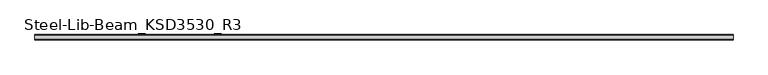
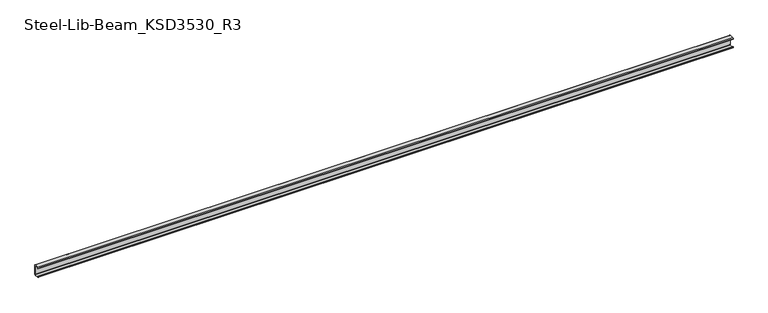
"""IFC4 building model written with IfcOpenShell, lengths in millimetres: beam geometry, Steel-Lib-Beam_KSD3530_R3 : BMS291_C-150×75x20x4.5."""

import ifcopenshell
import ifcopenshell.guid

model = None  # the IFC model being written
_history = None  # IfcOwnerHistory: only IFC2X3 demands one
_inside = {}  # id of a spatial element -> (the spatial element, [elements in it])
_under = {}  # id of a project, library or spatial element -> (it, [spatial elements below it])
_declared = {}  # id of a project -> (the project, [libraries it declares])
_typed = {}  # id of a type object -> (the type object, [elements of that type])
_made_of = {}  # id of a material, layer set ... -> (it, [elements and type objects made of it])


def new_model(schema):
    """Start an empty IFC model of exactly this schema.

    Asked for "IFC4X3", IfcOpenShell would pick the latest addendum, in which some entities
    have other attributes; the version numbers below select the first issue.
    IFC2X3 requires an IfcOwnerHistory on every rooted entity: one is made here for all.
    """
    global model, _history
    if schema == "IFC4X3":
        model = ifcopenshell.file(schema_version=(4, 3, 0, 0))
    else:
        model = ifcopenshell.file(schema=schema)
    _inside.clear()
    _under.clear()
    _declared.clear()
    _typed.clear()
    _made_of.clear()
    _history = None
    if model.schema == "IFC2X3":
        org = make("IfcOrganization", Name="unknown")
        user = make(
            "IfcPersonAndOrganization",
            ThePerson=make("IfcPerson", FamilyName="unknown"),
            TheOrganization=org,
        )
        app = make(
            "IfcApplication",
            ApplicationDeveloper=org,
            Version="unknown",
            ApplicationFullName="unknown",
            ApplicationIdentifier="unknown",
        )
        _history = make(
            "IfcOwnerHistory",
            OwningUser=user,
            OwningApplication=app,
            ChangeAction="ADDED",
            CreationDate=0,
        )
    return model


def make(cls, **values):
    """One entity of the class cls with the attributes given. An attribute that is None is left unset."""
    return model.create_entity(
        cls, **{name: value for name, value in values.items() if value is not None}
    )


def rooted(cls, **values):
    """An entity with a GlobalId (a new one), such as an element, a storey or a relation."""
    return make(cls, GlobalId=ifcopenshell.guid.new(), OwnerHistory=_history, **values)


def si_unit(unit_type, name, prefix=None):
    """IfcSIUnit, for example si_unit("LENGTHUNIT", "METRE", prefix="MILLI")."""
    return make("IfcSIUnit", UnitType=unit_type, Prefix=prefix, Name=name)


def assignment(units):
    """IfcUnitAssignment: the units of a project."""
    return None if units is None else make("IfcUnitAssignment", Units=units)


def point(xyz):
    """IfcCartesianPoint."""
    return None if xyz is None else make("IfcCartesianPoint", Coordinates=xyz)


def direction(xyz):
    """IfcDirection."""
    return None if xyz is None else make("IfcDirection", DirectionRatios=xyz)


def frame(location, z_axis=None, x_axis=None):
    """IfcAxis2Placement3D, a coordinate frame: its origin and axes. An axis left out is left unset."""
    return make(
        "IfcAxis2Placement3D",
        Location=point(location),
        Axis=direction(z_axis),
        RefDirection=direction(x_axis),
    )


def frame_2d(location, x_axis=None):
    """IfcAxis2Placement2D, a coordinate frame in the plane: its origin and x axis."""
    return make(
        "IfcAxis2Placement2D", Location=point(location), RefDirection=direction(x_axis)
    )


def origin():
    """The frame at (0, 0, 0) with its axes left unset."""
    return frame((0.0, 0.0, 0.0))


def place(relative_to, where):
    """IfcLocalPlacement: puts the frame where relative to a parent placement (None: the world)."""
    return make(
        "IfcLocalPlacement", PlacementRelTo=relative_to, RelativePlacement=where
    )


def context(
    kind, dimensions, precision=None, world=None, true_north=None, identifier=None
):
    """IfcGeometricRepresentationContext, for example the 3D "Model" context."""
    return make(
        "IfcGeometricRepresentationContext",
        ContextIdentifier=identifier,
        ContextType=kind,
        CoordinateSpaceDimension=dimensions,
        Precision=precision,
        WorldCoordinateSystem=world,
        TrueNorth=true_north,
    )


def project(units=None, contexts=None):
    """IfcProject with its units and contexts."""
    return rooted(
        "IfcProject",
        Name="project",
        RepresentationContexts=contexts,
        UnitsInContext=assignment(units),
    )


def spatial(cls, under=None, at=None, **own):
    """A site, building, storey or space (cls), placed at a placement, below another one or the project."""
    s = rooted(cls, ObjectPlacement=at, **own)
    if under is not None:
        _under.setdefault(under.id(), (under, []))[1].append(s)
    return s


def polyline(points):
    """IfcPolyline through the points."""
    return make("IfcPolyline", Points=[point(p) for p in points])


def circle_curve(where, radius):
    """IfcCircle in the frame where."""
    return make("IfcCircle", Position=where, Radius=radius)


def trimmed(basis, trim1, trim2, sense, master):
    """IfcTrimmedCurve: the piece of a basis curve between two trims."""
    return make(
        "IfcTrimmedCurve",
        BasisCurve=basis,
        Trim1=trim1,
        Trim2=trim2,
        SenseAgreement=sense,
        MasterRepresentation=master,
    )


def segment(curve, same_sense, transition):
    """IfcCompositeCurveSegment."""
    return make(
        "IfcCompositeCurveSegment",
        Transition=transition,
        SameSense=same_sense,
        ParentCurve=curve,
    )


def composite_curve(segments, self_intersect=None):
    """IfcCompositeCurve: segments joined end to end."""
    return make("IfcCompositeCurve", Segments=segments, SelfIntersect=self_intersect)


def outline(outer, holes=None, kind="AREA"):
    """IfcArbitraryClosedProfileDef: a profile drawn as a closed curve; with holes, ...WithVoids."""
    if holes is None:
        return make("IfcArbitraryClosedProfileDef", ProfileType=kind, OuterCurve=outer)
    return make(
        "IfcArbitraryProfileDefWithVoids",
        ProfileType=kind,
        OuterCurve=outer,
        InnerCurves=holes,
    )


def extrude(swept, where, along, depth):
    """IfcExtrudedAreaSolid: the profile swept, set in the frame where, extruded along a direction by depth."""
    return make(
        "IfcExtrudedAreaSolid",
        SweptArea=swept,
        Position=where,
        ExtrudedDirection=direction(along),
        Depth=depth,
    )


def shape(context_of_items, identifier, shape_type, items):
    """IfcShapeRepresentation: the items that make up one representation, for example the "Body"."""
    return make(
        "IfcShapeRepresentation",
        ContextOfItems=context_of_items,
        RepresentationIdentifier=identifier,
        RepresentationType=shape_type,
        Items=items,
    )


def source(mapping_origin, context_of_items, identifier, shape_type, items):
    """IfcRepresentationMap: a shape defined once, which mapped items show again and again."""
    return make(
        "IfcRepresentationMap",
        MappingOrigin=mapping_origin,
        MappedRepresentation=shape(context_of_items, identifier, shape_type, items),
    )


def transform(
    local_origin,
    x_axis=None,
    y_axis=None,
    z_axis=None,
    scale=None,
    scale2=None,
    scale3=None,
    uniform=True,
):
    """IfcCartesianTransformationOperator3D, or its non-uniform kind. x_axis, y_axis, z_axis: its Axis1, 2, 3."""
    if uniform:
        return make(
            "IfcCartesianTransformationOperator3D",
            Axis1=direction(x_axis),
            Axis2=direction(y_axis),
            LocalOrigin=point(local_origin),
            Scale=scale,
            Axis3=direction(z_axis),
        )
    return make(
        "IfcCartesianTransformationOperator3DnonUniform",
        Axis1=direction(x_axis),
        Axis2=direction(y_axis),
        LocalOrigin=point(local_origin),
        Scale=scale,
        Axis3=direction(z_axis),
        Scale2=scale2,
        Scale3=scale3,
    )


def mapped(mapping_source, mapping_target):
    """IfcMappedItem: shows the shape of a source again, moved by a transform."""
    return make(
        "IfcMappedItem", MappingSource=mapping_source, MappingTarget=mapping_target
    )


def made_of(thing, what):
    """Note that an element or type object is made of a material, layer set ...; save() writes the relation."""
    if what is not None:
        _made_of.setdefault(what.id(), (what, []))[1].append(thing)
    return thing


def element(
    cls,
    number,
    at=None,
    inside=None,
    cuts=None,
    type_object=None,
    material=None,
    context=None,
    identifier="Body",
    shape_type=None,
    held_by="IfcProductDefinitionShape",
    body=None,
    shapes=None,
    **own,
):
    """One element of the class cls, such as IfcWall. Its Tag is "e" and its number.

    at: its placement. inside: the storey or other place that contains it. cuts: it is an
    opening in that element (IfcRelVoidsElement). A single representation is given by context,
    identifier, shape_type and body (its items); several are given by shapes. held_by: the class
    of the entity that holds the representations. save() writes the other relations.
    """
    e = rooted(cls, Tag="e%d" % number, ObjectPlacement=at, **own)
    if body is not None:
        shapes = [shape(context, identifier, shape_type, body)]
    if shapes is not None:
        e.Representation = make(held_by, Representations=shapes)
    if inside is not None:
        _inside.setdefault(inside.id(), (inside, []))[1].append(e)
    if cuts is not None:
        rooted(
            "IfcRelVoidsElement", RelatingBuildingElement=cuts, RelatedOpeningElement=e
        )
    if type_object is not None:
        _typed.setdefault(type_object.id(), (type_object, []))[1].append(e)
    return made_of(e, material)


def aggregate(whole, parts):
    """IfcRelAggregates: a whole, such as a stair, and the parts it consists of."""
    return rooted("IfcRelAggregates", RelatingObject=whole, RelatedObjects=parts)


def save(model, path):
    """Write the relations noted so far, then the file.

    IfcRelAggregates (storeys below a building ...), IfcRelContainedInSpatialStructure (elements
    in a storey), IfcRelDefinesByType, IfcRelAssociatesMaterial and IfcRelDeclares: one each for
    every whole, place, type object, material and project.
    """
    for whole, parts in _under.values():
        aggregate(whole, parts)
    for where, things in _inside.values():
        rooted(
            "IfcRelContainedInSpatialStructure",
            RelatedElements=things,
            RelatingStructure=where,
        )
    for kind, things in _typed.values():
        rooted("IfcRelDefinesByType", RelatedObjects=things, RelatingType=kind)
    for what, things in _made_of.values():
        rooted("IfcRelAssociatesMaterial", RelatedObjects=things, RelatingMaterial=what)
    for by, libraries in _declared.values():
        rooted("IfcRelDeclares", RelatingContext=by, RelatedDefinitions=libraries)
    model.write(path)


def steel_lib_beam_ksd3530_r3_103558c8(model_context):
    return source(origin(), model_context, "Body", "SweptSolid", [
        extrude(outline(composite_curve([segment(trimmed(circle_curve(frame_2d((-41.0, 66.0)), 9.0), [point((-50.0, 66.0))], [point((-41.0, 75.0))], False, "CARTESIAN"), True, "CONTINUOUS"), segment(polyline([(-41.0, 75.0), (16.0, 75.0)]), True, "CONTINUOUS"), segment(trimmed(circle_curve(frame_2d((16.0, 66.0)), 9.0), [point((16.0, 75.0))], [point((25.0, 66.0))], False, "CARTESIAN"), True, "CONTINUOUS"), segment(polyline([(25.0, 66.0), (25.0, -66.0)]), True, "CONTINUOUS"), segment(trimmed(circle_curve(frame_2d((16.0, -66.0)), 9.0), [point((25.0, -66.0))], [point((16.0, -75.0))], False, "CARTESIAN"), True, "CONTINUOUS"), segment(polyline([(16.0, -75.0), (-41.0, -75.0)]), True, "CONTINUOUS"), segment(trimmed(circle_curve(frame_2d((-41.0, -66.0)), 9.0), [point((-41.0, -75.0))], [point((-50.0, -66.0))], False, "CARTESIAN"), True, "CONTINUOUS"), segment(polyline([(-50.0, -66.0), (-50.0, -55.0), (-45.5, -55.0), (-45.5, -66.0)]), True, "CONTINUOUS"), segment(trimmed(circle_curve(frame_2d((-41.0, -66.0)), 4.5), [point((-45.5, -66.0))], [point((-41.0, -70.5))], True, "CARTESIAN"), True, "CONTINUOUS"), segment(polyline([(-41.0, -70.5), (16.0, -70.5)]), True, "CONTINUOUS"), segment(trimmed(circle_curve(frame_2d((16.0, -66.0)), 4.5), [point((16.0, -70.5))], [point((20.5, -66.0))], True, "CARTESIAN"), True, "CONTINUOUS"), segment(polyline([(20.5, -66.0), (20.5, 66.0)]), True, "CONTINUOUS"), segment(trimmed(circle_curve(frame_2d((16.0, 66.0)), 4.5), [point((20.5, 66.0))], [point((16.0, 70.5))], True, "CARTESIAN"), True, "CONTINUOUS"), segment(polyline([(16.0, 70.5), (-41.0, 70.5)]), True, "CONTINUOUS"), segment(trimmed(circle_curve(frame_2d((-41.0, 66.0)), 4.5), [point((-41.0, 70.5))], [point((-45.5, 66.0))], True, "CARTESIAN"), True, "CONTINUOUS"), segment(polyline([(-45.5, 66.0), (-45.5, 55.0), (-50.0, 55.0), (-50.0, 66.0)]), True, "CONTINUOUS")], self_intersect=False)), frame((-4752.0, 0.0, 0.0), z_axis=(1.0, 0.0, 0.0), x_axis=(0.0, 1.0, 0.0)), (0.0, 0.0, 1.0), 9787.0),
    ])


if __name__ == "__main__":
    model = new_model("IFC4")
    model_context = context("Model", 3, world=origin())
    ifc_project = project(units=[si_unit("LENGTHUNIT", "METRE", prefix="MILLI")], contexts=[model_context])
    site = spatial("IfcSite", under=ifc_project)
    building = spatial("IfcBuilding", under=site)
    placement = place(None, origin())
    steel_lib_beam_ksd3530_r3_shape = steel_lib_beam_ksd3530_r3_103558c8(model_context)
    element("IfcBeam", 1, ObjectType="Steel-Lib-Beam_KSD3530_R3 : BMS291_C-150×75x20x4.5", at=placement, inside=building, context=model_context, shape_type="MappedRepresentation", body=[
        mapped(steel_lib_beam_ksd3530_r3_shape, transform((0.0, 0.0, 0.0), x_axis=(1.0, 0.0, 0.0), y_axis=(0.0, 1.0, 0.0), z_axis=(0.0, 0.0, 1.0))),
    ])
    save(model, "model.ifc")

# Revit data of these elements
# Type "Steel-Lib-Beam_KSD3530_R3 : BMS291_C-150×75x20x4.5"
#   Keynote = "C-150×75x20x4.5"
#   SteelWeight = "Light"
#   x = 0.0250 m
#   t1 = 0.0090 m
#   t = 0.0045 m
#   Surface Area = 0.629834 m²/m
#   Section Area = 13.9688 cm²
#   Mass per Unit Length = 10.9655 kg/m
#   C = 0.0200 m
#   A = 0.0750 m
#   Length [instance default] = 1.5000 m
#   H = 0.1500 m
#   hec_material4 [instance default] = none
#   hec_material3 [instance default] = none
#   hec_material2 [instance default] = none
#   hec_material1 [instance default] = none
#   Structural Material [instance default] = Metal - Steel - Light Gauge
#   Assembly Code = ""
# Element 1 (IfcBeam, "Steel-Lib-Beam_KSD3530_R3 : BMS291_C-150×75x20x4.5")
#   Structural Material = none
# Materials
#   "Metal - Steel - Light Gauge": class "Metal", colour RGB 247 247 247, transparency 0
